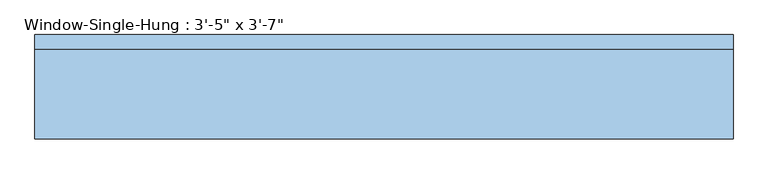
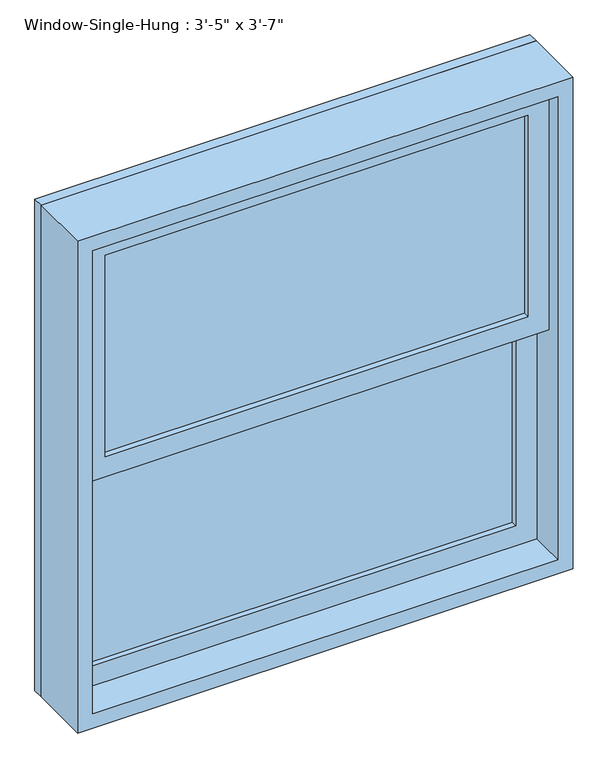
"""IFC4 building model written with IfcOpenShell, lengths in millimetres: window geometry."""

from ifc_helpers import new_model, si_unit, frame, origin, place, context, project, spatial, polyline, outline, extrude, source, transform, mapped, element, save


def window_8f49ead4(model_context):
    return source(origin(), model_context, "Body", "SweptSolid", [
        extrude(outline(polyline([(444.5, 1.5875), (-444.5, 1.5875), (-444.5, 7.9375), (444.5, 7.9375), (444.5, 1.5875)])), frame((0.0, 0.0, 990.6), z_axis=(0.0, 0.0, 1.0), x_axis=(1.0, 0.0, 0.0)), (0.0, 0.0, 1.0), 447.675),
        extrude(outline(polyline([(-444.5, 14.2875), (-444.5, 20.6375), (444.5, 20.6375), (444.5, 14.2875), (-444.5, 14.2875)])), frame((0.0, 0.0, 990.6), z_axis=(0.0, 0.0, 1.0), x_axis=(1.0, 0.0, 0.0)), (0.0, 0.0, 1.0), 447.675),
        extrude(outline(polyline([(444.5, -42.8625), (-444.5, -42.8625), (-444.5, -36.5125), (444.5, -36.5125), (444.5, -42.8625)])), frame((0.0, 0.0, 1482.725), z_axis=(0.0, 0.0, 1.0), x_axis=(1.0, 0.0, 0.0)), (0.0, 0.0, 1.0), 447.675),
        extrude(outline(polyline([(-444.5, -30.1625), (-444.5, -23.8125), (444.5, -23.8125), (444.5, -30.1625), (-444.5, -30.1625)])), frame((0.0, 0.0, 1482.725), z_axis=(0.0, 0.0, 1.0), x_axis=(1.0, 0.0, 0.0)), (0.0, 0.0, 1.0), 447.675),
        extrude(outline(polyline([(1482.725, 488.95), (1482.725, -488.95), (946.15, -488.95), (946.15, 488.95), (1482.725, 488.95)]), holes=[polyline([(1438.275, -444.5), (1438.275, 444.5), (990.6, 444.5), (990.6, -444.5), (1438.275, -444.5)])]), frame((0.0, -11.1125, 0.0), z_axis=(0.0, 1.0, 0.0), x_axis=(0.0, 0.0, 1.0)), (0.0, 0.0, 1.0), 44.45),
        extrude(outline(polyline([(1974.85, 488.95), (1974.85, -488.95), (1438.275, -488.95), (1438.275, 488.95), (1974.85, 488.95)]), holes=[polyline([(1930.4, -444.5), (1930.4, 444.5), (1482.725, 444.5), (1482.725, -444.5), (1930.4, -444.5)])]), frame((0.0, -55.5625, 0.0), z_axis=(0.0, 1.0, 0.0), x_axis=(0.0, 0.0, 1.0)), (0.0, 0.0, 1.0), 44.45),
        extrude(outline(polyline([(2006.6, 520.7), (2006.6, -520.7), (914.4, -520.7), (914.4, 520.7), (2006.6, 520.7)]), holes=[polyline([(1974.85, -488.95), (1974.85, 488.95), (946.15, 488.95), (946.15, -488.95), (1974.85, -488.95)])]), frame((0.0, -87.3125, 0.0), z_axis=(0.0, 1.0, 0.0), x_axis=(0.0, 0.0, 1.0)), (0.0, 0.0, 1.0), 133.35),
        extrude(outline(polyline([(2006.6, 520.7), (2006.6, -520.7), (914.4, -520.7), (914.4, 520.7), (2006.6, 520.7)]), holes=[polyline([(1987.55, 501.65), (933.45, 501.65), (933.45, -501.65), (1987.55, -501.65), (1987.55, 501.65)])]), frame((0.0, 46.0375, 0.0), z_axis=(0.0, 1.0, 0.0), x_axis=(0.0, 0.0, 1.0)), (0.0, 0.0, 1.0), 22.225),
    ])


if __name__ == "__main__":
    model = new_model("IFC4")
    model_context = context("Model", 3, world=origin())
    ifc_project = project(units=[si_unit("LENGTHUNIT", "METRE", prefix="MILLI")], contexts=[model_context])
    site = spatial("IfcSite", under=ifc_project)
    building = spatial("IfcBuilding", under=site)
    placement = place(None, origin())
    window_shape = window_8f49ead4(model_context)
    element("IfcWindow", 1, ObjectType="Window-Single-Hung : 3'-5\" x 3'-7\"", at=placement, inside=building, context=model_context, shape_type="MappedRepresentation", body=[
        mapped(window_shape, transform((0.0, 0.0, 0.0), x_axis=(1.0, 0.0, 0.0), y_axis=(0.0, 1.0, 0.0), z_axis=(0.0, 0.0, 1.0))),
    ])
    save(model, "model.ifc")

# Revit data of these elements
# Type "Window-Single-Hung : 3'-5\" x 3'-7\""
#   Type Mark = "25"
#   Fire Rating = "0.5h"
#   Construction Type Id = "DG-DR"
#   Assembly Code = "B2020100"
#   Analytic Construction = "Double glazing - domestic"
#   Wall Thickness [instance default] = 0' - 6"
#   Window Inset [instance default] = 0' - 0"
#   Visual Light Transmittance = 0.81
#   Thermal Resistance (R) = 0.319569 (m²·K)/W
#   Solar Heat Gain Coefficient = 0.76
#   Muntin Width = 2' - 11"
#   Muntin Height = 1' - 5 5/8"
#   Interior Wall Closure [instance default] = 0' - 1 1/2"
#   Rough Width = 3' - 5 1/2"
#   Rough Height = 3' - 7 1/2"
#   Frame Extension [instance default] = 0' - 1 1/4"
#   Exterior Wall Closure [instance default] = 0' - 0 1/2"
#   Extension Jamb [instance default] = 0' - 1 1/2"
#   Heat Transfer Coefficient (U) = 3.12929 W/(m²·K)
#   Height = 3' - 7"
#   Width = 3' - 5"
#   Top Muntin Visibility = yes
#   Indicator Visibility [instance default] = yes
#   Extension Jamb Visibility [instance default] = yes
#   Interior Trim Visibility [instance default] = yes
#   Exterior Trim Visibility [instance default] = yes
#   Bottom Muntin Visibility = yes
#   Muntin Pattern = Muntin Pattern_2x2 : Muntin Pattern_2x2
#   Interior Trim Material = Wood - Stained
#   Interior Trim = Trim-Window-Interior-Flat : Picture Frame
#   Exterior Trim Material = Clad - White
#   Exterior Trim = Trim-Window-Exterior-Flat : with Sill
#   Glass Panel Material = Glass
#   Exterior Frame Material = Clad - White
#   Interior Frame Material = Wood - Stained
#   Wall Closure = (empty or 0)
# Element 1 (IfcWindow, "Window-Single-Hung : 3'-5\" x 3'-7\"")
#   Wall Thickness = 0' - 5 3/8"
#   Extension Jamb = 0' - 0 7/8"
#   Materials on its faces: "Wood - Stained", "Glass", "Clad - White"
# Materials
#   "Wood - Stained": class "Wood", colour RGB 224 178 126, transparency 0, Cost = 0
#   "Clad - White": class "Wood", colour RGB 242 242 238, transparency 0, Cost = 0
#   "Glass": class "Glass", colour RGB 0 128 192, transparency 0.75, Description = "Soda Lime Glass", Cost = 0
